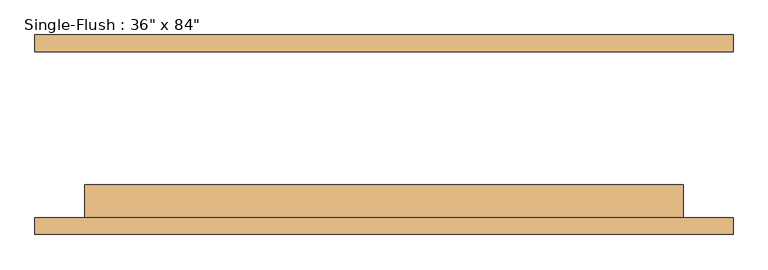
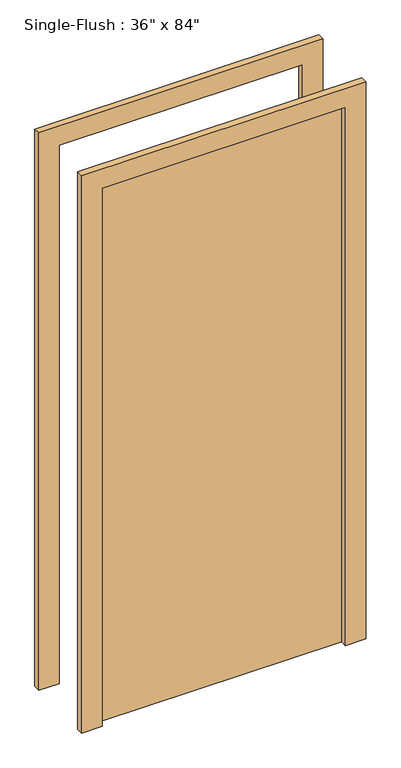
"""IFC4 building model written with IfcOpenShell, lengths in millimetres: door geometry."""

from ifc_helpers import new_model, si_unit, frame, origin, origin_with_axes, place, context, project, spatial, polyline, outline, extrude, source, transform, mapped, element, save


def door_9d8f1ff2(model_context):
    return source(origin(), model_context, "Body", "SweptSolid", [
        extrude(outline(polyline([(2209.8, -533.4), (0.0, -533.4), (0.0, -457.2), (2133.6, -457.2), (2133.6, 457.2), (0.0, 457.2), (0.0, 533.4), (2209.8, 533.4), (2209.8, -533.4)])), frame((0.0, -152.4, 0.0), z_axis=(0.0, 1.0, 0.0), x_axis=(0.0, 0.0, 1.0)), (0.0, 0.0, 1.0), 25.4),
        extrude(outline(polyline([(2209.8, 533.4), (2209.8, -533.4), (0.0, -533.4), (0.0, -457.2), (2133.6, -457.2), (2133.6, 457.2), (0.0, 457.2), (0.0, 533.4), (2209.8, 533.4)])), frame((0.0, 127.0, 0.0), z_axis=(0.0, 1.0, 0.0), x_axis=(0.0, 0.0, 1.0)), (0.0, 0.0, 1.0), 25.4),
        extrude(outline(polyline([(457.2, -76.2), (457.2, -127.0), (-457.2, -127.0), (-457.2, -76.2), (457.2, -76.2)])), origin_with_axes(), (0.0, 0.0, 1.0), 2133.6),
    ])


if __name__ == "__main__":
    model = new_model("IFC4")
    model_context = context("Model", 3, world=origin())
    ifc_project = project(units=[si_unit("LENGTHUNIT", "METRE", prefix="MILLI")], contexts=[model_context])
    site = spatial("IfcSite", under=ifc_project)
    building = spatial("IfcBuilding", under=site)
    placement = place(None, origin())
    door_shape = door_9d8f1ff2(model_context)
    element("IfcDoor", 1, ObjectType="Single-Flush : 36\" x 84\"", at=placement, inside=building, context=model_context, shape_type="MappedRepresentation", body=[
        mapped(door_shape, transform((0.0, 0.0, 0.0), x_axis=(1.0, 0.0, 0.0), y_axis=(0.0, 1.0, 0.0), z_axis=(0.0, 0.0, 1.0))),
    ])
    save(model, "model.ifc")

# Revit data of these elements
# Type "Single-Flush : 36\" x 84\""
#   Type Mark = "1"
#   Assembly Code = "C1020"
#   Thickness = 50.8 mm
#   Height = 2133.6 mm
#   Trim Projection Ext = 25.4 mm
#   Trim Projection Int = 25.4 mm
#   Trim Width = 76.2 mm
#   Width = 914.4 mm
#   Door Material = Door - Panel
#   Frame Material = Door - Frame
#   Function = (empty or 0)
#   Wall Closure = (empty or 0)
# Element 1 (IfcDoor, "Single-Flush : 36\" x 84\"")
#   Materials on its faces: "Door - Frame", "Door - Panel"
# Materials
#   "Door - Panel": class "Wood", colour RGB 210 159 95, transparency 0
#   "Door - Frame": class "Miscellaneous", colour RGB 118 70 51, transparency 0
